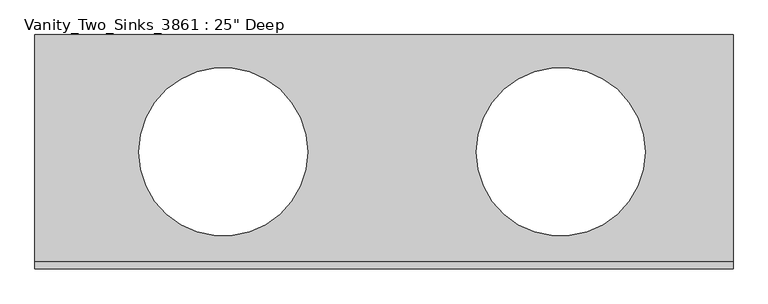
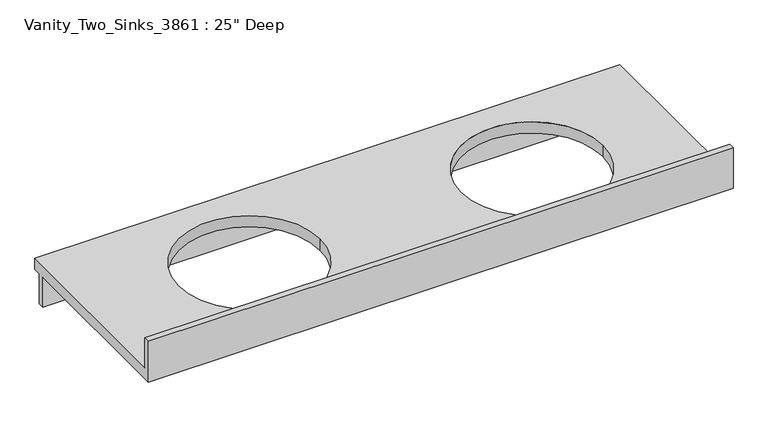
"""IFC4 building model written with IfcOpenShell, lengths in millimetres: furniture geometry."""

from ifc_helpers import new_model, si_unit, frame, origin, place, context, project, spatial, polyline, circle_curve, source, transform, mapped, element, save
from ifc_brep_helpers import plane_surface, revolved_surface, advanced_brep


def furniture_6b9eb554(model_context):
    return source(origin(), model_context, "Body", "AdvancedBrep", [
        advanced_brep(
        [(-1327.4622951, 635.0, 863.6), (-1327.4622951, 19.05, 863.6), (564.3712969, 19.05, 863.6), (564.3712969, 635.0, 863.6), (325.7362884, 317.5, 863.6), (-131.4637116, 317.5, 863.6), (-588.6637116, 317.5, 863.6), (-1045.8637116, 317.5, 863.6), (564.3712969, 635.0, 825.5), (564.3712969, 609.6, 825.5), (-1327.4622951, 609.6, 825.5), (-1327.4622951, 635.0, 825.5), (-1327.4622951, 0.0, 825.5), (-1327.4622951, 590.55, 825.5), (564.3712969, 590.55, 825.5), (564.3712969, 0.0, 825.5), (-131.4637116, 317.5, 825.5), (325.7362884, 317.5, 825.5), (-1045.8637116, 317.5, 825.5), (-588.6637116, 317.5, 825.5), (564.3712969, 0.0, 965.2), (-1327.4622951, 0.0, 965.2), (-1327.4622951, 609.6, 723.9), (-1327.4622951, 590.55, 723.9), (-1327.4622951, 19.05, 965.2), (564.3712969, 19.05, 965.2), (564.3712969, 590.55, 723.9), (564.3712969, 609.6, 723.9)],
        [
            (0, 1),
            (1, 2),
            (2, 3),
            (3, 0),
            (4, 5, circle_curve(frame((97.1362884, 317.5, 863.6), z_axis=(0.0, 0.0, -1.0), x_axis=(1.0, 0.0, 0.0)), 228.6)),
            (5, 4, circle_curve(frame((97.1362884, 317.5, 863.6), z_axis=(0.0, 0.0, -1.0), x_axis=(1.0, 0.0, 0.0)), 228.6)),
            (6, 7, circle_curve(frame((-817.2637116, 317.5, 863.6), z_axis=(0.0, 0.0, -1.0), x_axis=(1.0, 0.0, 0.0)), 228.6)),
            (7, 6, circle_curve(frame((-817.2637116, 317.5, 863.6), z_axis=(0.0, 0.0, -1.0), x_axis=(1.0, 0.0, 0.0)), 228.6)),
            (8, 9),
            (9, 10),
            (10, 11),
            (11, 8),
            (12, 13),
            (13, 14),
            (14, 15),
            (15, 12),
            (16, 17, circle_curve(frame((97.1362884, 317.5, 825.5), z_axis=(0.0, 0.0, 1.0), x_axis=(1.0, 0.0, 0.0)), 228.6)),
            (17, 16, circle_curve(frame((97.1362884, 317.5, 825.5), z_axis=(0.0, 0.0, 1.0), x_axis=(1.0, 0.0, 0.0)), 228.6)),
            (18, 19, circle_curve(frame((-817.2637116, 317.5, 825.5), z_axis=(0.0, 0.0, 1.0), x_axis=(1.0, 0.0, 0.0)), 228.6)),
            (19, 18, circle_curve(frame((-817.2637116, 317.5, 825.5), z_axis=(0.0, 0.0, 1.0), x_axis=(1.0, 0.0, 0.0)), 228.6)),
            (15, 20),
            (20, 21),
            (21, 12),
            (10, 22),
            (22, 23),
            (23, 13),
            (21, 24),
            (24, 1),
            (0, 11),
            (3, 8),
            (2, 25),
            (25, 20),
            (14, 26),
            (26, 27),
            (27, 9),
            (5, 16),
            (17, 4),
            (25, 24),
            (7, 18),
            (19, 6),
            (26, 23),
            (22, 27),
        ],
        [
            plane_surface(frame((-1327.4622951, 0.0, 863.6), z_axis=(0.0, 0.0, 1.0), x_axis=(-1.0, 0.0, 0.0))),
            plane_surface(frame((-1327.4622951, 0.0, 825.5), z_axis=(0.0, 0.0, -1.0), x_axis=(1.0, 0.0, 0.0))),
            plane_surface(frame((564.3712969, 0.0, 863.6), z_axis=(0.0, -1.0, 0.0), x_axis=(0.0, 0.0, -1.0))),
            plane_surface(frame((-1327.4622951, 0.0, 863.6), z_axis=(-1.0, 0.0, 0.0), x_axis=(0.0, 0.0, -1.0))),
            plane_surface(frame((-1327.4622951, 635.0, 863.6), z_axis=(0.0, 1.0, 0.0), x_axis=(0.0, 0.0, -1.0))),
            plane_surface(frame((564.3712969, 635.0, 863.6), z_axis=(1.0, 0.0, 0.0), x_axis=(0.0, 0.0, -1.0))),
            revolved_surface(polyline([(325.7362884, 317.5, 863.6), (325.7362884, 317.5, 825.5)]), (97.1362884, 317.5, 825.5), (0.0, 0.0, 1.0)),
            plane_surface(frame((-1327.4622951, 0.0, 965.2), z_axis=(0.0, 0.0, 1.0), x_axis=(0.0, 1.0, 0.0))),
            plane_surface(frame((-1327.4622951, 19.05, 965.2), z_axis=(0.0, 1.0, 0.0), x_axis=(0.0, 0.0, -1.0))),
            revolved_surface(polyline([(-588.6637115999999, 317.5, 863.6), (-588.6637115999999, 317.5, 825.5)]), (-817.2637116, 317.5, 825.5), (0.0, 0.0, 1.0)),
            plane_surface(frame((-1327.4622951, 590.55, 723.9), z_axis=(0.0, 0.0, -1.0), x_axis=(1.0, 0.0, 0.0))),
            plane_surface(frame((564.3712969, 590.55, 825.5), z_axis=(0.0, -1.0, 0.0), x_axis=(0.0, 0.0, -1.0))),
            plane_surface(frame((-1327.4622951, 609.6, 825.5), z_axis=(0.0, 1.0, 0.0), x_axis=(0.0, 0.0, -1.0))),
        ],
        [
            (0, [[1, 2, 3, 4], [5, 6], [7, 8]]),
            (1, [[9, 10, 11, 12]]),
            (1, [[13, 14, 15, 16], [17, 18], [19, 20]]),
            (2, [[21, 22, 23, -16]]),
            (3, [[-11, 24, 25, 26, -13, -23, 27, 28, -1, 29]]),
            (4, [[30, -12, -29, -4]]),
            (5, [[-3, 31, 32, -21, -15, 33, 34, 35, -9, -30]]),
            (6, [[-6, 36, -18, 37]]),
            (6, [[-17, -36, -5, -37]]),
            (7, [[-22, -32, 38, -27]]),
            (8, [[-31, -2, -28, -38]]),
            (9, [[-8, 39, -20, 40]]),
            (9, [[-19, -39, -7, -40]]),
            (10, [[41, -25, 42, -34]]),
            (11, [[-33, -14, -26, -41]]),
            (12, [[-24, -10, -35, -42]]),
        ],
    ),
    ])


if __name__ == "__main__":
    model = new_model("IFC4")
    model_context = context("Model", 3, world=origin())
    ifc_project = project(units=[si_unit("LENGTHUNIT", "METRE", prefix="MILLI")], contexts=[model_context])
    site = spatial("IfcSite", under=ifc_project)
    building = spatial("IfcBuilding", under=site)
    placement = place(None, origin())
    furniture_shape = furniture_6b9eb554(model_context)
    element("IfcFurniture", 1, ObjectType="Vanity_Two_Sinks_3861 : 25\" Deep", at=placement, inside=building, context=model_context, shape_type="MappedRepresentation", body=[
        mapped(furniture_shape, transform((0.0, 0.0, 0.0), x_axis=(1.0, 0.0, 0.0), y_axis=(0.0, 1.0, 0.0), z_axis=(0.0, 0.0, 1.0))),
    ])
    save(model, "model.ifc")

# Revit data of these elements
# Type "Vanity_Two_Sinks_3861 : 25\" Deep"
#   Assembly Code = "C1030400"
#   Sink Location Right [instance default] = 1' - 6"
#   Counter Thickness = 0' - 1 1/2"
#   Depth = 2' - 1"
#   Height = 2' - 10"
#   Length [instance default] = 6' - 0"
#   Sink Location Left [instance default] = 1' - 6"
#   Sink to Back Wall = 0' - 4"
#   Sink Opening Width [instance default] = 1' - 5"
#   Counter Top = Casework - Vanity Top
#   Width = 0
# Element 1 (IfcFurniture, "Vanity_Two_Sinks_3861 : 25\" Deep")
#   Sink Location Right = 1' - 6.39508"
#   Length = 6' - 2.48164"
#   Sink Location Left = 1' - 8.08656"
#   Materials on its faces: "Casework - Vanity Top"
# Materials
#   "Casework - Vanity Top": class "Unassigned", colour RGB 210 200 171, transparency 0, Comments = "Rendering appearance not upgraded "
